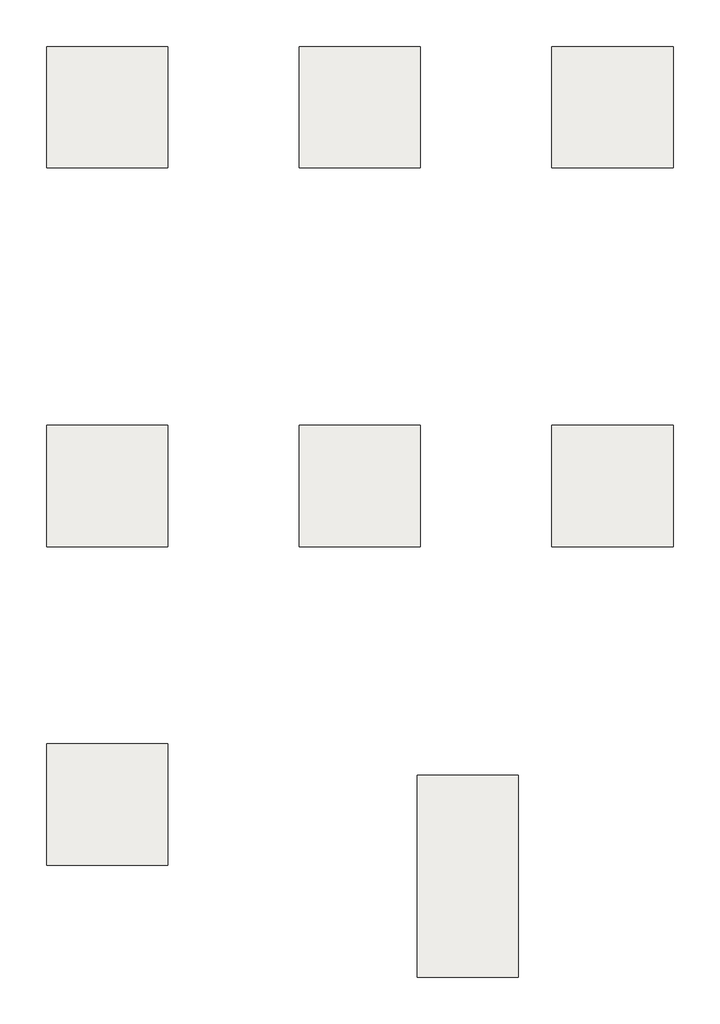
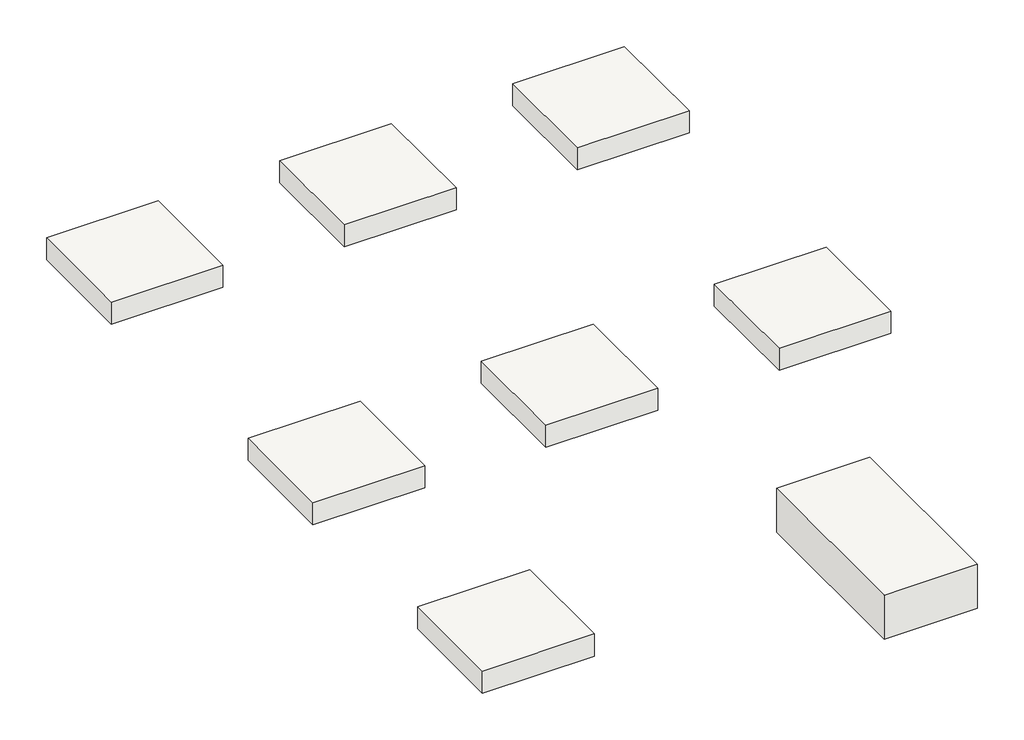
# Not in any storey: 8 slabs.
"""IFC4 building model written with IfcOpenShell, lengths in millimetres."""

import ifcopenshell
import ifcopenshell.guid

model = None  # the IFC model being written
_history = None  # IfcOwnerHistory: only IFC2X3 demands one
_inside = {}  # id of a spatial element -> (the spatial element, [elements in it])
_under = {}  # id of a project, library or spatial element -> (it, [spatial elements below it])
_declared = {}  # id of a project -> (the project, [libraries it declares])
_typed = {}  # id of a type object -> (the type object, [elements of that type])
_made_of = {}  # id of a material, layer set ... -> (it, [elements and type objects made of it])


def new_model(schema):
    """Start an empty IFC model of exactly this schema.

    Asked for "IFC4X3", IfcOpenShell would pick the latest addendum, in which some entities
    have other attributes; the version numbers below select the first issue.
    IFC2X3 requires an IfcOwnerHistory on every rooted entity: one is made here for all.
    """
    global model, _history
    if schema == "IFC4X3":
        model = ifcopenshell.file(schema_version=(4, 3, 0, 0))
    else:
        model = ifcopenshell.file(schema=schema)
    _inside.clear()
    _under.clear()
    _declared.clear()
    _typed.clear()
    _made_of.clear()
    _history = None
    if model.schema == "IFC2X3":
        org = make("IfcOrganization", Name="unknown")
        user = make(
            "IfcPersonAndOrganization",
            ThePerson=make("IfcPerson", FamilyName="unknown"),
            TheOrganization=org,
        )
        app = make(
            "IfcApplication",
            ApplicationDeveloper=org,
            Version="unknown",
            ApplicationFullName="unknown",
            ApplicationIdentifier="unknown",
        )
        _history = make(
            "IfcOwnerHistory",
            OwningUser=user,
            OwningApplication=app,
            ChangeAction="ADDED",
            CreationDate=0,
        )
    return model


def make(cls, **values):
    """One entity of the class cls with the attributes given. An attribute that is None is left unset."""
    return model.create_entity(
        cls, **{name: value for name, value in values.items() if value is not None}
    )


def rooted(cls, **values):
    """An entity with a GlobalId (a new one), such as an element, a storey or a relation."""
    return make(cls, GlobalId=ifcopenshell.guid.new(), OwnerHistory=_history, **values)


def si_unit(unit_type, name, prefix=None):
    """IfcSIUnit, for example si_unit("LENGTHUNIT", "METRE", prefix="MILLI")."""
    return make("IfcSIUnit", UnitType=unit_type, Prefix=prefix, Name=name)


def assignment(units):
    """IfcUnitAssignment: the units of a project."""
    return None if units is None else make("IfcUnitAssignment", Units=units)


def point(xyz):
    """IfcCartesianPoint."""
    return None if xyz is None else make("IfcCartesianPoint", Coordinates=xyz)


def direction(xyz):
    """IfcDirection."""
    return None if xyz is None else make("IfcDirection", DirectionRatios=xyz)


def frame(location, z_axis=None, x_axis=None):
    """IfcAxis2Placement3D, a coordinate frame: its origin and axes. An axis left out is left unset."""
    return make(
        "IfcAxis2Placement3D",
        Location=point(location),
        Axis=direction(z_axis),
        RefDirection=direction(x_axis),
    )


def origin():
    """The frame at (0, 0, 0) with its axes left unset."""
    return frame((0.0, 0.0, 0.0))


def place(relative_to, where):
    """IfcLocalPlacement: puts the frame where relative to a parent placement (None: the world)."""
    return make(
        "IfcLocalPlacement", PlacementRelTo=relative_to, RelativePlacement=where
    )


def context(
    kind, dimensions, precision=None, world=None, true_north=None, identifier=None
):
    """IfcGeometricRepresentationContext, for example the 3D "Model" context."""
    return make(
        "IfcGeometricRepresentationContext",
        ContextIdentifier=identifier,
        ContextType=kind,
        CoordinateSpaceDimension=dimensions,
        Precision=precision,
        WorldCoordinateSystem=world,
        TrueNorth=true_north,
    )


def project(units=None, contexts=None):
    """IfcProject with its units and contexts."""
    return rooted(
        "IfcProject",
        Name="project",
        RepresentationContexts=contexts,
        UnitsInContext=assignment(units),
    )


def spatial(cls, under=None, at=None, **own):
    """A site, building, storey or space (cls), placed at a placement, below another one or the project."""
    s = rooted(cls, ObjectPlacement=at, **own)
    if under is not None:
        _under.setdefault(under.id(), (under, []))[1].append(s)
    return s


def polyline(points):
    """IfcPolyline through the points."""
    return make("IfcPolyline", Points=[point(p) for p in points])


def outline(outer, holes=None, kind="AREA"):
    """IfcArbitraryClosedProfileDef: a profile drawn as a closed curve; with holes, ...WithVoids."""
    if holes is None:
        return make("IfcArbitraryClosedProfileDef", ProfileType=kind, OuterCurve=outer)
    return make(
        "IfcArbitraryProfileDefWithVoids",
        ProfileType=kind,
        OuterCurve=outer,
        InnerCurves=holes,
    )


def extrude(swept, where, along, depth):
    """IfcExtrudedAreaSolid: the profile swept, set in the frame where, extruded along a direction by depth."""
    return make(
        "IfcExtrudedAreaSolid",
        SweptArea=swept,
        Position=where,
        ExtrudedDirection=direction(along),
        Depth=depth,
    )


def shape(context_of_items, identifier, shape_type, items):
    """IfcShapeRepresentation: the items that make up one representation, for example the "Body"."""
    return make(
        "IfcShapeRepresentation",
        ContextOfItems=context_of_items,
        RepresentationIdentifier=identifier,
        RepresentationType=shape_type,
        Items=items,
    )


def source(mapping_origin, context_of_items, identifier, shape_type, items):
    """IfcRepresentationMap: a shape defined once, which mapped items show again and again."""
    return make(
        "IfcRepresentationMap",
        MappingOrigin=mapping_origin,
        MappedRepresentation=shape(context_of_items, identifier, shape_type, items),
    )


def transform(
    local_origin,
    x_axis=None,
    y_axis=None,
    z_axis=None,
    scale=None,
    scale2=None,
    scale3=None,
    uniform=True,
):
    """IfcCartesianTransformationOperator3D, or its non-uniform kind. x_axis, y_axis, z_axis: its Axis1, 2, 3."""
    if uniform:
        return make(
            "IfcCartesianTransformationOperator3D",
            Axis1=direction(x_axis),
            Axis2=direction(y_axis),
            LocalOrigin=point(local_origin),
            Scale=scale,
            Axis3=direction(z_axis),
        )
    return make(
        "IfcCartesianTransformationOperator3DnonUniform",
        Axis1=direction(x_axis),
        Axis2=direction(y_axis),
        LocalOrigin=point(local_origin),
        Scale=scale,
        Axis3=direction(z_axis),
        Scale2=scale2,
        Scale3=scale3,
    )


def mapped(mapping_source, mapping_target):
    """IfcMappedItem: shows the shape of a source again, moved by a transform."""
    return make(
        "IfcMappedItem", MappingSource=mapping_source, MappingTarget=mapping_target
    )


def made_of(thing, what):
    """Note that an element or type object is made of a material, layer set ...; save() writes the relation."""
    if what is not None:
        _made_of.setdefault(what.id(), (what, []))[1].append(thing)
    return thing


def element(
    cls,
    number,
    at=None,
    inside=None,
    cuts=None,
    type_object=None,
    material=None,
    context=None,
    identifier="Body",
    shape_type=None,
    held_by="IfcProductDefinitionShape",
    body=None,
    shapes=None,
    **own,
):
    """One element of the class cls, such as IfcWall. Its Tag is "e" and its number.

    at: its placement. inside: the storey or other place that contains it. cuts: it is an
    opening in that element (IfcRelVoidsElement). A single representation is given by context,
    identifier, shape_type and body (its items); several are given by shapes. held_by: the class
    of the entity that holds the representations. save() writes the other relations.
    """
    e = rooted(cls, Tag="e%d" % number, ObjectPlacement=at, **own)
    if body is not None:
        shapes = [shape(context, identifier, shape_type, body)]
    if shapes is not None:
        e.Representation = make(held_by, Representations=shapes)
    if inside is not None:
        _inside.setdefault(inside.id(), (inside, []))[1].append(e)
    if cuts is not None:
        rooted(
            "IfcRelVoidsElement", RelatingBuildingElement=cuts, RelatedOpeningElement=e
        )
    if type_object is not None:
        _typed.setdefault(type_object.id(), (type_object, []))[1].append(e)
    return made_of(e, material)


def aggregate(whole, parts):
    """IfcRelAggregates: a whole, such as a stair, and the parts it consists of."""
    return rooted("IfcRelAggregates", RelatingObject=whole, RelatedObjects=parts)


def save(model, path):
    """Write the relations noted so far, then the file.

    IfcRelAggregates (storeys below a building ...), IfcRelContainedInSpatialStructure (elements
    in a storey), IfcRelDefinesByType, IfcRelAssociatesMaterial and IfcRelDeclares: one each for
    every whole, place, type object, material and project.
    """
    for whole, parts in _under.values():
        aggregate(whole, parts)
    for where, things in _inside.values():
        rooted(
            "IfcRelContainedInSpatialStructure",
            RelatedElements=things,
            RelatingStructure=where,
        )
    for kind, things in _typed.values():
        rooted("IfcRelDefinesByType", RelatedObjects=things, RelatingType=kind)
    for what, things in _made_of.values():
        rooted("IfcRelAssociatesMaterial", RelatedObjects=things, RelatingMaterial=what)
    for by, libraries in _declared.values():
        rooted("IfcRelDeclares", RelatingContext=by, RelatedDefinitions=libraries)
    model.write(path)


def ft211_2400x2400x500_5fe39465(model_context):
    return source(origin(), model_context, "Body", "SweptSolid", [
        extrude(outline(polyline([(1200.0, 1200.0), (1200.0, -1200.0), (-1200.0, -1200.0), (-1200.0, 1200.0), (1200.0, 1200.0)])), frame((0.0, 0.0, -500.0), z_axis=(0.0, 0.0, 1.0), x_axis=(1.0, 0.0, 0.0)), (0.0, 0.0, 1.0), 500.0),
    ])


model = new_model("IFC4")

# Units and contexts
model_context = context("Model", 3, world=origin())
ifc_project = project(units=[si_unit("LENGTHUNIT", "METRE", prefix="MILLI")], contexts=[model_context])

# Site, building
site = spatial("IfcSite", under=ifc_project)
building = spatial("IfcBuilding", under=site)

# Slabs
placement = place(None, origin())
element("IfcSlab", 1, ObjectType="FT211-Footing-Rectangular_더미삭제 : FT211_2400x2400x500", at=placement, inside=building, context=model_context, shape_type="SweptSolid", body=[
    extrude(outline(polyline([(11200.0, 22199.5208589), (11200.0, 19799.5208589), (8800.0, 19799.5208589), (8800.0, 22199.5208589), (11200.0, 22199.5208589)])), frame((0.0, 0.0, -1800.0), z_axis=(0.0, 0.0, 1.0), x_axis=(1.0, 0.0, 0.0)), (0.0, 0.0, 1.0), 500.0),
])
element("IfcSlab", 2, ObjectType="FT211-Footing-Rectangular_더미삭제 : FT211_2400x2400x500", at=placement, inside=building, context=model_context, shape_type="SweptSolid", body=[
    extrude(outline(polyline([(6200.0, 22199.5208589), (6200.0, 19799.5208589), (3800.0, 19799.5208589), (3800.0, 22199.5208589), (6200.0, 22199.5208589)])), frame((0.0, 0.0, -1800.0), z_axis=(0.0, 0.0, 1.0), x_axis=(1.0, 0.0, 0.0)), (0.0, 0.0, 1.0), 500.0),
])
element("IfcSlab", 3, ObjectType="FT211-Footing-Rectangular_더미삭제 : FT211_2400x2400x500", at=placement, inside=building, context=model_context, shape_type="SweptSolid", body=[
    extrude(outline(polyline([(1200.0, 22199.5208589), (1200.0, 19799.5208589), (-1200.0, 19799.5208589), (-1200.0, 22199.5208589), (1200.0, 22199.5208589)])), frame((0.0, 0.0, -1800.0), z_axis=(0.0, 0.0, 1.0), x_axis=(1.0, 0.0, 0.0)), (0.0, 0.0, 1.0), 500.0),
])
element("IfcSlab", 4, ObjectType="FT211-Footing-Rectangular_더미삭제 : FT211_2400x2400x500", at=placement, inside=building, context=model_context, shape_type="SweptSolid", body=[
    extrude(outline(polyline([(1200.0, 14699.5208589), (1200.0, 12299.5208589), (-1200.0, 12299.5208589), (-1200.0, 14699.5208589), (1200.0, 14699.5208589)])), frame((0.0, 0.0, -1800.0), z_axis=(0.0, 0.0, 1.0), x_axis=(1.0, 0.0, 0.0)), (0.0, 0.0, 1.0), 500.0),
])
ft211_2400x2400x500_shape = ft211_2400x2400x500_5fe39465(model_context)
element("IfcSlab", 5, ObjectType="FT211-Footing-Rectangular_더미삭제 : FT211_2400x2400x500", at=placement, inside=building, context=model_context, shape_type="MappedRepresentation", body=[
    mapped(ft211_2400x2400x500_shape, transform((5000.0, 13499.5208589, -1300.0), x_axis=(1.0, 0.0, 0.0), y_axis=(0.0, 1.0, 0.0), z_axis=(0.0, 0.0, 1.0))),
])
element("IfcSlab", 6, ObjectType="FT211-Footing-Rectangular_더미삭제 : FT211_2400x2400x500", at=placement, inside=building, context=model_context, shape_type="MappedRepresentation", body=[
    mapped(ft211_2400x2400x500_shape, transform((10000.0, 13499.5208589, -1300.0), x_axis=(1.0, 0.0, 0.0), y_axis=(0.0, 1.0, 0.0), z_axis=(0.0, 0.0, 1.0))),
])
element("IfcSlab", 7, ObjectType="FT211-Footing-Rectangular_더미삭제 : FT211_2400x2400x500 new", at=placement, inside=building, context=model_context, shape_type="SweptSolid", body=[
    extrude(outline(polyline([(1200.0, 8399.5208589), (1200.0, 5999.5208589), (-1200.0, 5999.5208589), (-1200.0, 8399.5208589), (1200.0, 8399.5208589)])), frame((0.0, 0.0, -1800.0), z_axis=(0.0, 0.0, 1.0), x_axis=(1.0, 0.0, 0.0)), (0.0, 0.0, 1.0), 500.0),
])
element("IfcSlab", 8, ObjectType="FT211-Footing-Rectangular_더미삭제 : FT211_4000x2000x1000 new", at=placement, inside=building, context=model_context, shape_type="SweptSolid", body=[
    extrude(outline(polyline([(8135.1052251, 7774.5208589), (8135.1052251, 3774.5208589), (6135.1052251, 3774.5208589), (6135.1052251, 7774.5208589), (8135.1052251, 7774.5208589)])), frame((0.0, 0.0, -1800.0), z_axis=(0.0, 0.0, 1.0), x_axis=(1.0, 0.0, 0.0)), (0.0, 0.0, 1.0), 1000.0),
])

save(model, "model.ifc")

# Revit data of these elements
# Project information
#   Building Name = "MAIN GATE SECURITY BUILDING"
#   Project Status = "Project Status"
#   Client Name = "현대엔지니어링"
#   Project Address = "서울시 종로구 율곡로 75(계동)"
#   Project Name = "Therma Visayas Energy Project"
#   Project Number = "-"
# Grids (mm)
#   "A": line (0, 24502.793) -> (0, 11308.625)
#   "B": line (5000, 24502.793) -> (5000, 11308.625)
#   "C": line (10000, 24502.793) -> (10000, 11308.625)
#   "1": line (-3860.098, 13499.521) -> (12441.468, 13499.521)
#   "2": line (-3860.098, 20999.521) -> (12441.468, 20999.521)
# Type "FT211-Footing-Rectangular_더미삭제 : FT211_2400x2400x500"
#   Top bar = "D25@300"
#   Description = "UG Shallow Foundation"
#   Bottom bar = "D20@300"
#   Width = 2400 mm
#   Length = 2400 mm
#   Foundation Thickness = 500 mm
#   Structural Material [instance default] = A03AC032-00007_Structural Concrete_Type1_25MPa-30Mpa
#   Assembly Code = ""
# Type "FT211-Footing-Rectangular_더미삭제 : FT211_2400x2400x500 new"
#   Top bar = "D25@300"
#   Description = "UG Shallow Foundation"
#   Bottom bar = "D20@300"
#   Width = 2400 mm
#   Length = 2400 mm
#   Foundation Thickness = 500 mm
#   Structural Material [instance default] = A03AC032-00007_Structural Concrete_Type1_25MPa-30Mpa
#   Assembly Code = ""
# Type "FT211-Footing-Rectangular_더미삭제 : FT211_4000x2000x1000 new"
#   Top bar = "D25@300"
#   Description = "UG Shallow Foundation"
#   Bottom bar = "D20@300"
#   Width = 2000 mm
#   Length = 4000 mm
#   Foundation Thickness = 1000 mm
#   Structural Material [instance default] = A03AC032-00007_Structural Concrete_Type1_25MPa-30Mpa
#   Assembly Code = ""
# Elements 1, 2, 3, 4, 5, 6 (IfcSlab, "FT211-Footing-Rectangular_더미삭제 : FT211_2400x2400x500")
#   Comments = ""
#   Mark = "F1"
#   F01) Building Name = "Main Gate House"
#   F11) Project Building Tag_Type-1 = "Common"
#   F12) Project Building Tag_Type-2 = "Common"
#   F13) Project Facility Code = "Facility Code"
#   F21) Structural Type = "Concrete"
#   F31) Standard Building Code = "IBC"
#   F41) Discipline = "AR"
#   F51) Plan Start Date-Engineering = "2015-01-01"
#   F52) Plan Finish Date-Engineering = "2015-12-31"
#   F53) Duration = "365"
#   F54) Actual Start Date-Engineering = "2015-01-01"
#   F55) Actual Finish Date-Engineering = "2015-12-31"
#   F61) Plan Start Date-Construction = "2016-08-19"
#   F62) Plan Finish Date-Construction = "2017-01-31"
#   F64) Actual Start Date-Construction = "2016-08-19"
#   F63) Duration = "202"
#   F65) Actual Finish Date-Construction = "2017-01-31"
#   F91) Plant Type = "CFPP"
#   F92) KKS Structures, Building = "UYF"
#   P01) Project Name = "TVEP"
#   P02) Project Configuration = "CFB Boiler x 2(Foster Wheeler) + STG x 2(Alstom, 150MW)"
#   P03) Project Abbreviation = "TVEP"
#   P04) Project Code = "BEPH1402"
#   P05) Project Stage = "In operation"
#   P06) Project Location = "Sito Looc, Barangay Bato, Toledo City in Philippines"
#   P07) Project Owner = "Therma Visayas, Inc."
#   P08) Project O.E = "Flour"
#   P09) Project Schedule = "ITB Issueing Date : 2013.07.30\r\nSite Survey : 2013.08.19-20\r\nBid Closing Date : 2013.11.29\r\nPreferred Bidder Notice 접수 : 2014.04.27\r\nTarget award date : 2014 05\r\nLOA 접수 : 2014.05.21\r\nSigning Ceremony : 2014.05.30"
#   P10) Basic Wind Speed = "55.6 m/s"
#   P11) Seismic = "NSCP 2010, Zone 4 (PGA : 0.4g)"
#   P12) Soil = "Sc"
#   P13) Soil Capacity = "100kN/m2"
#   P14) Pile Capacity = "PHC(D400) : 1200kN"
#   W00) Work Master Code = "A03AC032-00007"
#   W01) Work Master_Lv1 = "Concrete Work"
#   W02) Work Master_Lv2 = "Substructure Work"
#   W03) Work Master_Spec.1 = "Cement Type-1"
#   W04) Work Master_Spec.2 = "25MPa < F'c (Cylinder Strength) ≤ 30MPa"
#   W11) Activity ID = "C02AGB010"
#   W12) Activity Name = "Main Gate Security Building - Building Foundation"
#   W13) Plan Start Date = "2016-08-19"
#   W14) Plan Finish Date = "2016-09-22"
#   W15) Duration = "26"
#   W16) Actual Start Date = "2016-08-19"
#   W17) Actual Finish Date = "2016-09-22"
#   R02) Unit Price = 0
#   Structural Material = A03AC032-00007_Structural Concrete_Type1_25MPa-30Mpa
#   Phase Created = New Construction
#   Materials on its faces: "A03AC032-00007_Structural Concrete_Type1_25MPa-30Mpa"
# Element 7 (IfcSlab, "FT211-Footing-Rectangular_더미삭제 : FT211_2400x2400x500 new")
#   Comments = ""
#   F01) Building Name = "Main Gate House"
#   F11) Project Building Tag_Type-1 = "Common"
#   F12) Project Building Tag_Type-2 = "Common"
#   F13) Project Facility Code = "Facility Code"
#   F21) Structural Type = "Concrete"
#   F31) Standard Building Code = "IBC"
#   F41) Discipline = "AR"
#   F51) Plan Start Date-Engineering = "2015-01-01"
#   F52) Plan Finish Date-Engineering = "2015-12-31"
#   F53) Duration = "365"
#   F54) Actual Start Date-Engineering = "2015-01-01"
#   F55) Actual Finish Date-Engineering = "2015-12-31"
#   F61) Plan Start Date-Construction = "2016-08-19"
#   F62) Plan Finish Date-Construction = "2017-01-31"
#   F64) Actual Start Date-Construction = "2016-08-19"
#   F63) Duration = "202"
#   F65) Actual Finish Date-Construction = "2017-01-31"
#   F91) Plant Type = "CFPP"
#   F92) KKS Structures, Building = "UYF"
#   P01) Project Name = "TVEP"
#   P02) Project Configuration = "CFB Boiler x 2(Foster Wheeler) + STG x 2(Alstom, 150MW)"
#   P03) Project Abbreviation = "TVEP"
#   P04) Project Code = "BEPH1402"
#   P05) Project Stage = "In operation"
#   P06) Project Location = "Sito Looc, Barangay Bato, Toledo City in Philippines"
#   P07) Project Owner = "Therma Visayas, Inc."
#   P08) Project O.E = "Flour"
#   P09) Project Schedule = "ITB Issueing Date : 2013.07.30\r\nSite Survey : 2013.08.19-20\r\nBid Closing Date : 2013.11.29\r\nPreferred Bidder Notice 접수 : 2014.04.27\r\nTarget award date : 2014 05\r\nLOA 접수 : 2014.05.21\r\nSigning Ceremony : 2014.05.30"
#   P10) Basic Wind Speed = "55.6 m/s"
#   P11) Seismic = "NSCP 2010, Zone 4 (PGA : 0.4g)"
#   P12) Soil = "Sc"
#   P13) Soil Capacity = "100kN/m2"
#   P14) Pile Capacity = "PHC(D400) : 1200kN"
#   W00) Work Master Code = "A03AC032-00007"
#   W01) Work Master_Lv1 = "Concrete Work"
#   W02) Work Master_Lv2 = "Substructure Work"
#   W03) Work Master_Spec.1 = "Cement Type-1"
#   W04) Work Master_Spec.2 = "25MPa < F'c (Cylinder Strength) ≤ 30MPa"
#   W11) Activity ID = "C02AGB010"
#   W12) Activity Name = "Main Gate Security Building - Building Foundation"
#   W13) Plan Start Date = "2016-08-19"
#   W14) Plan Finish Date = "2016-09-22"
#   W15) Duration = "26"
#   W16) Actual Start Date = "2016-08-19"
#   W17) Actual Finish Date = "2016-09-22"
#   R02) Unit Price = 0
#   Structural Material = A03AC032-00007_Structural Concrete_Type1_25MPa-30Mpa
#   Phase Created = New Construction
#   Materials on its faces: "A03AC032-00007_Structural Concrete_Type1_25MPa-30Mpa"
# Element 8 (IfcSlab, "FT211-Footing-Rectangular_더미삭제 : FT211_4000x2000x1000 new")
#   Comments = ""
#   F01) Building Name = "Main Gate House"
#   F11) Project Building Tag_Type-1 = "Common"
#   F12) Project Building Tag_Type-2 = "Common"
#   F13) Project Facility Code = "Facility Code"
#   F21) Structural Type = "Concrete"
#   F31) Standard Building Code = "IBC"
#   F41) Discipline = "AR"
#   F51) Plan Start Date-Engineering = "2015-01-01"
#   F52) Plan Finish Date-Engineering = "2015-12-31"
#   F53) Duration = "365"
#   F54) Actual Start Date-Engineering = "2015-01-01"
#   F55) Actual Finish Date-Engineering = "2015-12-31"
#   F61) Plan Start Date-Construction = "2016-08-19"
#   F62) Plan Finish Date-Construction = "2017-01-31"
#   F64) Actual Start Date-Construction = "2016-08-19"
#   F63) Duration = "202"
#   F65) Actual Finish Date-Construction = "2017-01-31"
#   F91) Plant Type = "CFPP"
#   F92) KKS Structures, Building = "UYF"
#   P01) Project Name = "TVEP"
#   P02) Project Configuration = "CFB Boiler x 2(Foster Wheeler) + STG x 2(Alstom, 150MW)"
#   P03) Project Abbreviation = "TVEP"
#   P04) Project Code = "BEPH1402"
#   P05) Project Stage = "In operation"
#   P06) Project Location = "Sito Looc, Barangay Bato, Toledo City in Philippines"
#   P07) Project Owner = "Therma Visayas, Inc."
#   P08) Project O.E = "Flour"
#   P09) Project Schedule = "ITB Issueing Date : 2013.07.30\r\nSite Survey : 2013.08.19-20\r\nBid Closing Date : 2013.11.29\r\nPreferred Bidder Notice 접수 : 2014.04.27\r\nTarget award date : 2014 05\r\nLOA 접수 : 2014.05.21\r\nSigning Ceremony : 2014.05.30"
#   P10) Basic Wind Speed = "55.6 m/s"
#   P11) Seismic = "NSCP 2010, Zone 4 (PGA : 0.4g)"
#   P12) Soil = "Sc"
#   P13) Soil Capacity = "100kN/m2"
#   P14) Pile Capacity = "PHC(D400) : 1200kN"
#   W00) Work Master Code = "A03AC032-00007"
#   W01) Work Master_Lv1 = "Concrete Work"
#   W02) Work Master_Lv2 = "Substructure Work"
#   W03) Work Master_Spec.1 = "Cement Type-1"
#   W04) Work Master_Spec.2 = "25MPa < F'c (Cylinder Strength) ≤ 30MPa"
#   W11) Activity ID = "C02AGB010"
#   W12) Activity Name = "Main Gate Security Building - Building Foundation"
#   W13) Plan Start Date = "2016-08-19"
#   W14) Plan Finish Date = "2016-09-22"
#   W15) Duration = "26"
#   W16) Actual Start Date = "2016-08-19"
#   W17) Actual Finish Date = "2016-09-22"
#   R02) Unit Price = 0
#   Structural Material = A03AC032-00007_Structural Concrete_Type1_25MPa-30Mpa
#   Phase Created = New Construction
#   Materials on its faces: "A03AC032-00007_Structural Concrete_Type1_25MPa-30Mpa"
# Materials
#   "A03AC032-00007_Structural Concrete_Type1_25MPa-30Mpa": class "Concrete", colour RGB 176 176 176, transparency 0, Keynote = "09910.A1", Description = "Reinf. Conc.", W00) Work Master Code = "A03AC032-00007", W01) Work Master_Lv1 = "Concrete Work", W02) Work Master_Lv2 = "Substructure Work", W03) Work Master_Spec.1 = "Structural Concrete", W04) Work Master_Spec.2 = "Cement Type-1", W05) Work Master_Spec.3 = "25MPa < F'c (Cylinder Strength) ≤ 30MPa", Cost = 0
